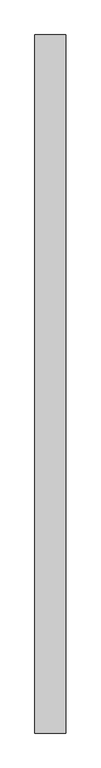
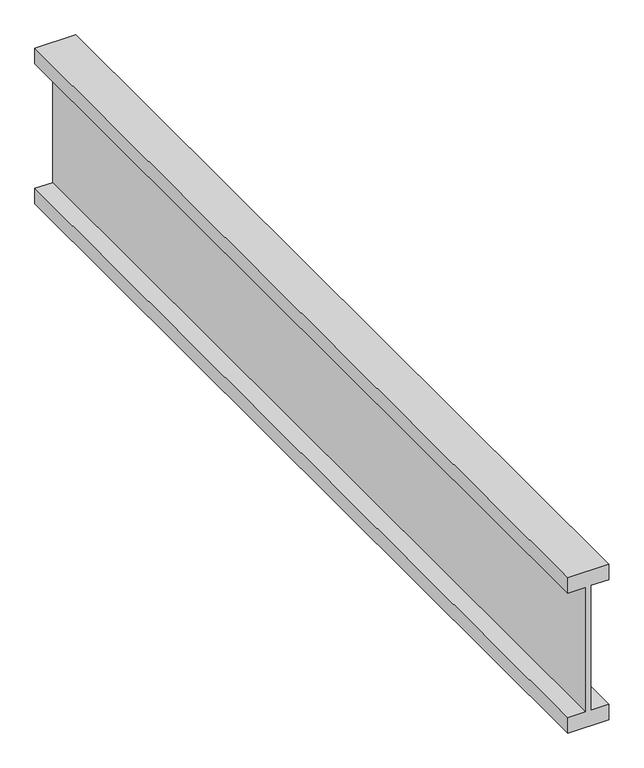
"""IFC4 building model written with IfcOpenShell, lengths in millimetres: proxy geometry, Framing065 7730 : Framing065 7730."""

from ifc_helpers import new_model, si_unit, frame, origin, place, context, project, spatial, polyline, outline, extrude, source, transform, mapped, element, save


def generic_models_252a1c86(model_context):
    return source(origin(), model_context, "Body", "SweptSolid", [
        extrude(outline(polyline([(40077.771, 8096.295938), (39792.021, 8096.295938), (39792.021, 8057.402188), (39757.096, 8057.402188), (39757.096, 8146.302188), (39792.021, 8146.302188), (39792.021, 8107.408438), (40077.771, 8107.408438), (40077.771, 8146.302188), (40112.696, 8146.302188), (40112.696, 8057.402188), (40077.771, 8057.402188), (40077.771, 8096.295938)])), frame((0.0, -3747.9491938, 0.0), z_axis=(0.0, 1.0, 0.0), x_axis=(0.0, 0.0, 1.0)), (0.0, 0.0, 1.0), 2000.0),
    ])


if __name__ == "__main__":
    model = new_model("IFC4")
    model_context = context("Model", 3, world=origin())
    ifc_project = project(units=[si_unit("LENGTHUNIT", "METRE", prefix="MILLI")], contexts=[model_context])
    site = spatial("IfcSite", under=ifc_project)
    building = spatial("IfcBuilding", under=site)
    placement = place(None, origin())
    generic_models_shape = generic_models_252a1c86(model_context)
    element("IfcBuildingElementProxy", 1, Name="Framing065 7730 : Framing065 7730", ObjectType="Framing065 7730 : Framing065 7730", at=placement, inside=building, context=model_context, shape_type="MappedRepresentation", body=[
        mapped(generic_models_shape, transform((0.0, 0.0, 0.0), x_axis=(1.0, 0.0, 0.0), y_axis=(0.0, 1.0, 0.0), z_axis=(0.0, 0.0, 1.0))),
    ])
    save(model, "model.ifc")

# Revit data of these elements
# Type "Framing065 7730 : Framing065 7730"
#   NameOverride = "Framing065"
# Element 1 (IfcBuildingElementProxy, "Framing065 7730 : Framing065 7730")
#   Materials on its faces: "WOOD FRAMING (SEE STRUCT DWGS)"
# Materials
#   "WOOD FRAMING (SEE STRUCT DWGS)": class "Unassigned", colour RGB 224 188 168, transparency 0, Cost = 0
